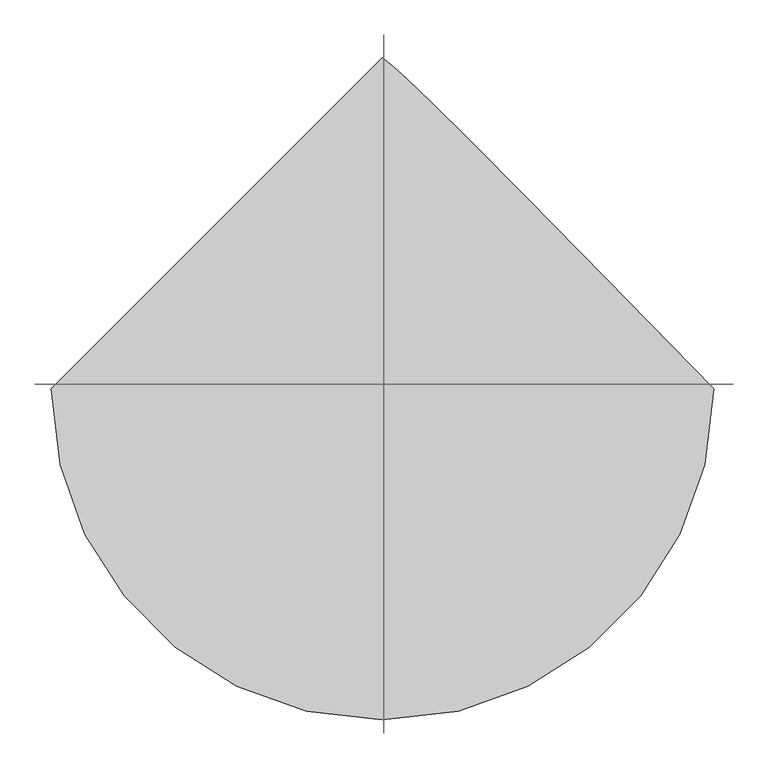
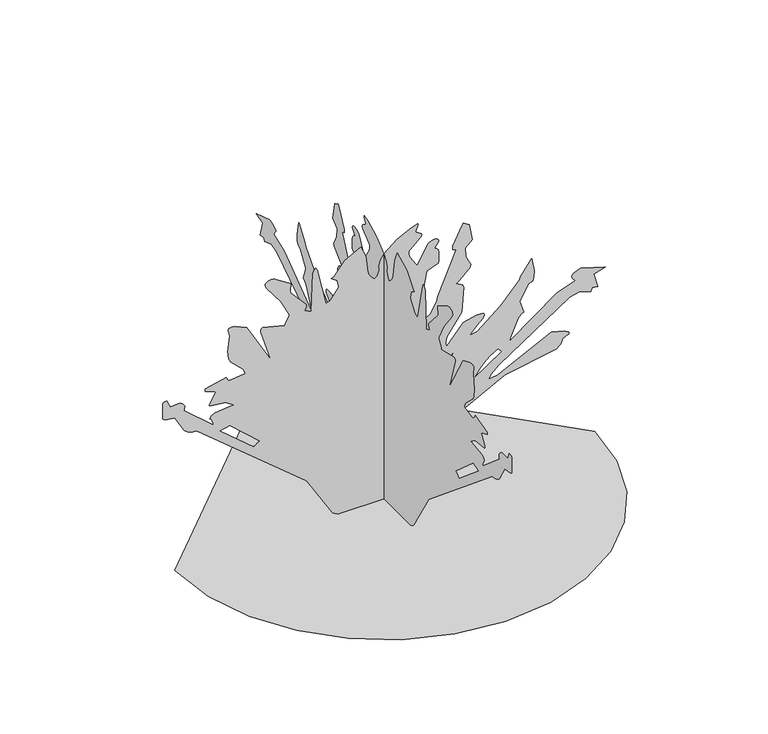
"""IFC4 building model written with IfcOpenShell, lengths in millimetres: proxy geometry, prairie dropseed 26760 : prairie dropseed 26760."""

import ifcopenshell
import ifcopenshell.guid

model = None  # the IFC model being written
_history = None  # IfcOwnerHistory: only IFC2X3 demands one
_inside = {}  # id of a spatial element -> (the spatial element, [elements in it])
_under = {}  # id of a project, library or spatial element -> (it, [spatial elements below it])
_declared = {}  # id of a project -> (the project, [libraries it declares])
_typed = {}  # id of a type object -> (the type object, [elements of that type])
_made_of = {}  # id of a material, layer set ... -> (it, [elements and type objects made of it])


def new_model(schema):
    """Start an empty IFC model of exactly this schema.

    Asked for "IFC4X3", IfcOpenShell would pick the latest addendum, in which some entities
    have other attributes; the version numbers below select the first issue.
    IFC2X3 requires an IfcOwnerHistory on every rooted entity: one is made here for all.
    """
    global model, _history
    if schema == "IFC4X3":
        model = ifcopenshell.file(schema_version=(4, 3, 0, 0))
    else:
        model = ifcopenshell.file(schema=schema)
    _inside.clear()
    _under.clear()
    _declared.clear()
    _typed.clear()
    _made_of.clear()
    _history = None
    if model.schema == "IFC2X3":
        org = make("IfcOrganization", Name="unknown")
        user = make(
            "IfcPersonAndOrganization",
            ThePerson=make("IfcPerson", FamilyName="unknown"),
            TheOrganization=org,
        )
        app = make(
            "IfcApplication",
            ApplicationDeveloper=org,
            Version="unknown",
            ApplicationFullName="unknown",
            ApplicationIdentifier="unknown",
        )
        _history = make(
            "IfcOwnerHistory",
            OwningUser=user,
            OwningApplication=app,
            ChangeAction="ADDED",
            CreationDate=0,
        )
    return model


def make(cls, **values):
    """One entity of the class cls with the attributes given. An attribute that is None is left unset."""
    return model.create_entity(
        cls, **{name: value for name, value in values.items() if value is not None}
    )


def rooted(cls, **values):
    """An entity with a GlobalId (a new one), such as an element, a storey or a relation."""
    return make(cls, GlobalId=ifcopenshell.guid.new(), OwnerHistory=_history, **values)


def si_unit(unit_type, name, prefix=None):
    """IfcSIUnit, for example si_unit("LENGTHUNIT", "METRE", prefix="MILLI")."""
    return make("IfcSIUnit", UnitType=unit_type, Prefix=prefix, Name=name)


def assignment(units):
    """IfcUnitAssignment: the units of a project."""
    return None if units is None else make("IfcUnitAssignment", Units=units)


def point(xyz):
    """IfcCartesianPoint."""
    return None if xyz is None else make("IfcCartesianPoint", Coordinates=xyz)


def direction(xyz):
    """IfcDirection."""
    return None if xyz is None else make("IfcDirection", DirectionRatios=xyz)


def frame(location, z_axis=None, x_axis=None):
    """IfcAxis2Placement3D, a coordinate frame: its origin and axes. An axis left out is left unset."""
    return make(
        "IfcAxis2Placement3D",
        Location=point(location),
        Axis=direction(z_axis),
        RefDirection=direction(x_axis),
    )


def origin():
    """The frame at (0, 0, 0) with its axes left unset."""
    return frame((0.0, 0.0, 0.0))


def place(relative_to, where):
    """IfcLocalPlacement: puts the frame where relative to a parent placement (None: the world)."""
    return make(
        "IfcLocalPlacement", PlacementRelTo=relative_to, RelativePlacement=where
    )


def context(
    kind, dimensions, precision=None, world=None, true_north=None, identifier=None
):
    """IfcGeometricRepresentationContext, for example the 3D "Model" context."""
    return make(
        "IfcGeometricRepresentationContext",
        ContextIdentifier=identifier,
        ContextType=kind,
        CoordinateSpaceDimension=dimensions,
        Precision=precision,
        WorldCoordinateSystem=world,
        TrueNorth=true_north,
    )


def project(units=None, contexts=None):
    """IfcProject with its units and contexts."""
    return rooted(
        "IfcProject",
        Name="project",
        RepresentationContexts=contexts,
        UnitsInContext=assignment(units),
    )


def spatial(cls, under=None, at=None, **own):
    """A site, building, storey or space (cls), placed at a placement, below another one or the project."""
    s = rooted(cls, ObjectPlacement=at, **own)
    if under is not None:
        _under.setdefault(under.id(), (under, []))[1].append(s)
    return s


def point_list(points):
    """IfcCartesianPointList2D or 3D."""
    cls = (
        "IfcCartesianPointList2D" if len(points[0]) == 2 else "IfcCartesianPointList3D"
    )
    return make(cls, CoordList=points)


def triangles(points, corners, closed=None, point_numbers=None):
    """IfcTriangulatedFaceSet: each triangle names its three corners, points numbered from 1."""
    return make(
        "IfcTriangulatedFaceSet",
        Coordinates=point_list(points),
        Closed=closed,
        CoordIndex=corners,
        PnIndex=point_numbers,
    )


def shape(context_of_items, identifier, shape_type, items):
    """IfcShapeRepresentation: the items that make up one representation, for example the "Body"."""
    return make(
        "IfcShapeRepresentation",
        ContextOfItems=context_of_items,
        RepresentationIdentifier=identifier,
        RepresentationType=shape_type,
        Items=items,
    )


def source(mapping_origin, context_of_items, identifier, shape_type, items):
    """IfcRepresentationMap: a shape defined once, which mapped items show again and again."""
    return make(
        "IfcRepresentationMap",
        MappingOrigin=mapping_origin,
        MappedRepresentation=shape(context_of_items, identifier, shape_type, items),
    )


def transform(
    local_origin,
    x_axis=None,
    y_axis=None,
    z_axis=None,
    scale=None,
    scale2=None,
    scale3=None,
    uniform=True,
):
    """IfcCartesianTransformationOperator3D, or its non-uniform kind. x_axis, y_axis, z_axis: its Axis1, 2, 3."""
    if uniform:
        return make(
            "IfcCartesianTransformationOperator3D",
            Axis1=direction(x_axis),
            Axis2=direction(y_axis),
            LocalOrigin=point(local_origin),
            Scale=scale,
            Axis3=direction(z_axis),
        )
    return make(
        "IfcCartesianTransformationOperator3DnonUniform",
        Axis1=direction(x_axis),
        Axis2=direction(y_axis),
        LocalOrigin=point(local_origin),
        Scale=scale,
        Axis3=direction(z_axis),
        Scale2=scale2,
        Scale3=scale3,
    )


def mapped(mapping_source, mapping_target):
    """IfcMappedItem: shows the shape of a source again, moved by a transform."""
    return make(
        "IfcMappedItem", MappingSource=mapping_source, MappingTarget=mapping_target
    )


def made_of(thing, what):
    """Note that an element or type object is made of a material, layer set ...; save() writes the relation."""
    if what is not None:
        _made_of.setdefault(what.id(), (what, []))[1].append(thing)
    return thing


def element(
    cls,
    number,
    at=None,
    inside=None,
    cuts=None,
    type_object=None,
    material=None,
    context=None,
    identifier="Body",
    shape_type=None,
    held_by="IfcProductDefinitionShape",
    body=None,
    shapes=None,
    **own,
):
    """One element of the class cls, such as IfcWall. Its Tag is "e" and its number.

    at: its placement. inside: the storey or other place that contains it. cuts: it is an
    opening in that element (IfcRelVoidsElement). A single representation is given by context,
    identifier, shape_type and body (its items); several are given by shapes. held_by: the class
    of the entity that holds the representations. save() writes the other relations.
    """
    e = rooted(cls, Tag="e%d" % number, ObjectPlacement=at, **own)
    if body is not None:
        shapes = [shape(context, identifier, shape_type, body)]
    if shapes is not None:
        e.Representation = make(held_by, Representations=shapes)
    if inside is not None:
        _inside.setdefault(inside.id(), (inside, []))[1].append(e)
    if cuts is not None:
        rooted(
            "IfcRelVoidsElement", RelatingBuildingElement=cuts, RelatedOpeningElement=e
        )
    if type_object is not None:
        _typed.setdefault(type_object.id(), (type_object, []))[1].append(e)
    return made_of(e, material)


def aggregate(whole, parts):
    """IfcRelAggregates: a whole, such as a stair, and the parts it consists of."""
    return rooted("IfcRelAggregates", RelatingObject=whole, RelatedObjects=parts)


def save(model, path):
    """Write the relations noted so far, then the file.

    IfcRelAggregates (storeys below a building ...), IfcRelContainedInSpatialStructure (elements
    in a storey), IfcRelDefinesByType, IfcRelAssociatesMaterial and IfcRelDeclares: one each for
    every whole, place, type object, material and project.
    """
    for whole, parts in _under.values():
        aggregate(whole, parts)
    for where, things in _inside.values():
        rooted(
            "IfcRelContainedInSpatialStructure",
            RelatedElements=things,
            RelatingStructure=where,
        )
    for kind, things in _typed.values():
        rooted("IfcRelDefinesByType", RelatedObjects=things, RelatingType=kind)
    for what, things in _made_of.values():
        rooted("IfcRelAssociatesMaterial", RelatedObjects=things, RelatingMaterial=what)
    for by, libraries in _declared.values():
        rooted("IfcRelDeclares", RelatingContext=by, RelatedDefinitions=libraries)
    model.write(path)


def entourage_02fa341a(model_context):
    return source(origin(), model_context, "Body", "Tessellation", [
        triangles([(-1145.8724991, 0.0, 0.0001203), (-1115.5778366, -262.5577928, 0.0001203), (-1029.3040329, -503.6753972, 0.0001203), (-893.9573524, -716.4439871, 0.0001203), (-716.4439871, -893.9573524, 0.0001203), (-503.6753972, -1029.3040329, 0.0001203), (-262.5577928, -1115.5778366, 0.0001203), (5.01e-05, -1145.8724991, 0.0001203), (262.5577928, -1115.5778366, 0.0001203), (503.6753972, -1029.3040329, 0.0001203), (716.4439871, -893.9573524, 0.0001203), (893.9573524, -716.4439871, 0.0001203), (1029.3040329, -503.6753972, 0.0001203), (1115.5778366, -262.5577928, 0.0001203), (1145.8724991, 0.0001002, 0.0001203), (773.4874529, 381.9735961, 0.0001203), (497.4218908, 663.2029781, 0.0001203), (301.6205247, 860.4800354, 0.0001203), (170.0304827, 990.5943317, 0.0001203), (86.5989292, 1070.3377928, 0.0001203), (35.272797, 1116.4998734, 0.0001203), (-0.0001503, 1145.8724991, 0.0001203), (191.5793673, 16.4808481, 1518.7299728), (190.2057411, 16.4808481, 1512.532386), (177.5557501, 16.4808481, 1485.8293648), (178.0462362, 16.4808481, 1480.5131195), (207.8564987, 16.4808481, 1461.7196445), (211.32233, 16.4808481, 1451.7881287), (204.1071818, 16.4808481, 1439.5808796), (144.6111222, 16.4808481, 1389.2583698), (141.1229358, 16.4808481, 1381.6383408), (140.426721, 16.4808481, 1366.2256187), (146.0929631, 16.4808481, 1347.6911396), (178.4658327, 16.4808481, 1296.2230602), (186.7823127, 16.4808481, 1288.0619305), (190.0609643, 16.4808481, 1288.211776), (245.3213086, 16.4808481, 1386.9849621), (252.3454438, 16.4808481, 1394.9860725), (265.8470906, 16.4808481, 1400.4698948), (281.8237317, 16.4808481, 1402.5959278), (289.4335869, 16.4808481, 1401.7577522), (296.0960073, 16.4808481, 1399.3065937), (301.2827002, 16.4808481, 1394.9860725), (303.525532, 16.4808481, 1388.0517574), (301.6992627, 16.4808481, 1380.2565937), (279.0398718, 16.4808481, 1350.4953289), (292.1132926, 16.4808481, 1346.2916611), (300.5334, 16.4808481, 1335.2070179), (305.1155694, 16.4808481, 1319.5453285), (303.9395511, 16.4808481, 1268.0670753), (301.2827002, 16.4808481, 1257.0687641), (238.9982207, 16.4808481, 1234.823465), (219.7373687, 16.4808742, 1135.2349216), (208.8420127, 16.4808742, 1067.5641249), (212.3832936, 16.4808742, 1036.2585503), (225.652015, 16.4808742, 1007.9299015), (234.5499094, 16.4808742, 967.8917931), (248.2595922, 16.4808742, 970.7670536), (258.6512544, 16.4808742, 978.4505962), (292.3850601, 16.4808742, 1039.0729134), (298.2194605, 16.4808742, 1065.3949986), (399.1592477, 16.4808481, 1301.557037), (381.5697327, 16.4808481, 1309.1974136), (379.2862601, 16.4808481, 1328.9001354), (432.7863739, 16.4808481, 1431.8338234), (439.1998996, 16.4808481, 1439.4742001), (469.1567193, 16.4808481, 1422.9108215), (470.340368, 16.4808481, 1421.67892), (488.1381915, 16.4808481, 1328.2525005), (448.0975396, 16.4808481, 1292.6593243), (452.5450879, 16.4808481, 1243.7211777), (475.4661089, 16.4808742, 1195.1663652), (479.2405515, 16.4808742, 1190.3352648), (474.884422, 16.4808742, 1175.0165051), (415.7048584, 16.4808742, 1116.6548058), (399.1592477, 16.4808742, 1105.8064854), (400.510546, 16.4808742, 1104.4069342), (434.7498078, 16.4808742, 1083.5611135), (441.3436641, 16.4808742, 1069.7841202), (428.4937943, 16.4808742, 930.2133516), (347.4472878, 16.4808992, 815.783563), (341.366518, 16.4808992, 788.9789492), (345.7734438, 16.4808992, 758.7935097), (439.1998996, 16.4808742, 865.5651175), (512.8727283, 16.4808742, 883.5687424), (542.821954, 16.4808742, 883.172473), (547.2034452, 16.4808742, 881.851696), (550.2463918, 16.4808742, 879.4843987), (551.976119, 16.4808742, 876.1493551), (552.4231484, 16.4808742, 871.9304266), (551.610371, 16.4808742, 866.9087854), (549.5681992, 16.4808742, 861.1709089), (543.2842441, 16.4808742, 853.7287033), (531.917714, 16.4808742, 842.4993742), (517.6733437, 16.4808992, 828.930653), (502.7584474, 16.4808992, 814.4704165), (489.3751436, 16.4808992, 800.5638525), (479.7282034, 16.4808992, 788.6613813), (476.0198178, 16.4808992, 780.210807), (513.8201632, 16.4808992, 789.5783312), (642.9667133, 16.4808742, 892.3291815), (746.172187, 16.4808742, 1007.9299015), (749.7891901, 16.4808742, 1021.8363928), (808.727453, 16.4808742, 1102.2682566), (812.905759, 16.4808742, 1105.8064854), (824.3001944, 16.4808742, 1031.1582075), (823.6322119, 16.4808742, 994.8412382), (817.3558508, 16.4808742, 972.3393414), (795.110479, 16.4808742, 967.8917931), (747.0028049, 16.4808742, 882.9210348), (746.172187, 16.4808742, 878.9128492), (768.4175589, 16.4808992, 812.1793499), (753.3274189, 16.4808992, 805.8165842), (738.2855318, 16.4808992, 789.0373032), (695.1587311, 16.4808992, 686.8503719), (692.7864195, 16.4808992, 669.8145658), (947.0688635, 16.4808742, 860.4216087), (1048.699506, 16.4808742, 896.7081293), (1031.5646507, 16.4808742, 917.3609385), (1030.2641487, 16.4808742, 922.2631102), (1030.9016825, 16.4808742, 927.8511412), (1034.3306883, 16.4808742, 934.1604944), (1040.9118273, 16.4808742, 940.3403498), (1059.8323294, 16.4808742, 950.6222803), (1080.2666925, 16.4808742, 955.3314405), (1088.7376144, 16.4808742, 954.5440613), (1213.3071184, 16.4808742, 914.5034094), (1151.0236382, 16.4808742, 896.7081293), (1173.2664665, 16.4808992, 816.6268982), (1142.1259981, 16.4808992, 821.0769899), (1133.2283581, 16.4808992, 803.2817099), (1073.0276722, 16.4808742, 824.1351608), (1018.2448242, 16.4808992, 810.9525352), (631.9609171, 16.4808992, 554.5135732), (591.7932381, 16.4808992, 516.5074991), (577.1145555, 16.4808992, 491.8592943), (627.4016024, 16.4808992, 498.6258508), (914.8336218, 16.4808992, 642.3291796), (919.6799829, 16.4808992, 643.1216457), (989.570775, 16.4808992, 625.9969643), (1013.5077587, 16.4808992, 611.3792519), (1017.1018707, 16.4808992, 604.5339211), (1013.9115858, 16.4808992, 600.0584312), (1009.2633957, 16.4808992, 596.634476), (980.9245731, 16.4808992, 585.3568577), (971.1252439, 16.4808992, 556.8427915), (945.85215, 16.4808992, 537.2669515), (663.4595032, 16.4808992, 486.10365), (303.2308916, 16.4809242, 297.9146645), (169.4772643, 16.4809242, 161.3263992), (69.2098062, 16.4809242, 12.9610616), (67.9149089, 16.4809242, 9.6154435), (64.4996195, 16.4809242, 6.7499111), (47.3677937, 16.4809242, 1.1487808), (-237.5664222, 16.4809242, 3.55e-05), (-244.2689927, 16.4809242, 1.6405105), (-251.0271739, 16.4809242, 4.0836423), (-257.5565174, 16.4809242, 7.0952757), (-263.5737918, 16.4809242, 10.4413515), (-268.793495, 16.4809242, 13.8879604), (-272.9311604, 16.4809242, 17.2006602), (-275.702303, 16.4809242, 20.1455931), (-415.6845471, 16.4809242, 251.3398547), (-1015.5905531, 16.4808992, 749.8933262), (-1043.5331789, 16.4808992, 753.4493591), (-1066.7030582, 16.4808992, 763.3172161), (-1085.8064707, 16.4808992, 778.3058361), (-1135.7099653, 16.4808742, 865.5651175), (-1188.5954, 16.4808742, 874.7803253), (-1197.2085371, 16.4808742, 878.409973), (-1202.4434647, 16.4808742, 883.3603975), (-1200.9524946, 16.4808742, 970.6299253), (-1197.9959164, 16.4808742, 976.7894331), (-1180.2006363, 16.4808742, 981.2369814), (-1162.4053562, 16.4808742, 941.1963295), (-1112.0319775, 16.4808742, 943.6424011), (-1102.0192892, 16.4808742, 939.9618845), (-1092.2453945, 16.4808742, 932.1361267), (-1082.3241251, 16.4808742, 918.9535011), (-1086.0451916, 16.4808742, 894.3433754), (-1086.7716734, 16.4808742, 892.2580376), (-926.6116093, 16.4808992, 754.3434179), (-925.605784, 16.4808992, 759.362443), (-927.0764791, 16.4808992, 766.1722017), (-938.5826809, 16.4808992, 788.0010292), (-942.1971405, 16.4808992, 792.6314152), (-944.4068893, 16.4808992, 794.3840698), (-937.4142929, 16.4808992, 808.8823854), (-919.3421402, 16.4808992, 818.6817146), (-823.4569319, 16.4808742, 829.6215265), (-815.3899097, 16.4808742, 829.97463), (-858.7680759, 16.4808742, 860.6984814), (-944.4068893, 16.4808742, 870.0152092), (-947.1628258, 16.4808742, 873.2892826), (-945.4203449, 16.4808742, 881.8338919), (-918.6309191, 16.4808742, 930.5131153), (-913.2664209, 16.4808742, 936.7487812), (-916.3169615, 16.4808742, 939.0652822), (-971.1023529, 16.4808742, 963.4417013), (-971.1023529, 16.4808742, 976.7894331), (-855.4305616, 16.4808742, 1003.4823532), (-846.5329216, 16.4808742, 985.6870731), (-841.8745577, 16.4808742, 979.8552343), (-829.7383799, 16.4808742, 977.9705383), (-753.1064295, 16.4808742, 990.1346214), (-756.4770086, 16.4808742, 1006.0553793), (-765.4127277, 16.4808742, 1020.5536949), (-831.3791954, 16.4808742, 1083.2842409), (-840.7899582, 16.4808742, 1103.5102592), (-847.4701464, 16.4808742, 1148.4429817), (-835.9664881, 16.4808481, 1236.4922585), (-844.9453732, 16.4808481, 1268.2270947), (-844.5237419, 16.4808481, 1274.356081), (-842.0828299, 16.4808481, 1279.3142086), (-823.4467581, 16.4808481, 1281.6536007), (-807.3482494, 16.4808481, 1280.2336292), (-744.2087894, 16.4808481, 1252.618745), (-611.5748068, 16.4808742, 1020.9982172), (-667.4397108, 16.4808742, 1200.5004147), (-666.7716557, 16.4808742, 1209.9873356), (-663.0404154, 16.4808742, 1217.4803375), (-655.2298456, 16.4808742, 1221.4783493), (-535.1105061, 16.4808742, 1190.3352648), (-533.8786045, 16.4808742, 1199.9263218), (-512.8651342, 16.4808481, 1239.2736294), (-511.3157375, 16.4808481, 1244.1986195), (-557.3532981, 16.4808481, 1337.1500679), (-634.6126448, 16.4808481, 1439.0804741), (-643.7160135, 16.4808481, 1457.800407), (-641.8821138, 16.4808481, 1466.1671928), (-637.6073021, 16.4808481, 1471.8948956), (-632.047249, 16.4808481, 1476.1239979), (-625.5575289, 16.4808481, 1478.9915554), (-611.2090588, 16.4808481, 1481.1760151), (-597.39395, 16.4808481, 1479.5149246), (-503.9674942, 16.4808481, 1421.67892), (-502.3393596, 16.4808481, 1414.2646923), (-507.1602862, 16.4808481, 1383.6296436), (-506.7665603, 16.4808481, 1375.9283695), (-503.9674942, 16.4808481, 1368.290609), (-419.4386421, 16.4808481, 1270.4164959), (-417.9679833, 16.4808481, 1265.4483398), (-418.4759829, 16.4808481, 1259.8959171), (-428.3362822, 16.4808481, 1239.2736294), (-392.7457583, 16.4808742, 1221.4783493), (-382.6517524, 16.4808481, 1438.78587), (-376.0604396, 16.4808481, 1454.3636982), (-366.0502948, 16.4808481, 1461.7196445), (-358.5369452, 16.4808481, 1448.6461693), (-312.6644546, 16.4808481, 1243.7211777), (-312.6644546, 16.4808481, 1239.2736294), (-297.8790925, 16.4808481, 1242.0853764), (-285.9918639, 16.4808481, 1249.6164574), (-241.4823532, 16.4808481, 1310.4546043), (-250.3804838, 16.4808481, 1350.4953289), (-281.5214609, 16.4808481, 1372.7406281), (-269.5834359, 16.4808481, 1376.9621727), (-207.497836, 16.4808481, 1449.829818), (-121.3619509, 16.4808481, 1497.3102047), (-95.2247926, 16.4808481, 1437.6657349), (-83.2026885, 16.4808481, 1344.1731857), (-76.9446311, 16.4808481, 1324.6506855), (-65.1584955, 16.4808481, 1306.0909172), (-45.7307615, 16.4808481, 1288.211776), (-41.5217161, 16.4808481, 1290.5004444), (-35.9095768, 16.4808481, 1296.6929443), (-29.9423425, 16.4808481, 1305.7657917), (-24.6679461, 16.4808481, 1316.7005894), (-21.135356, 16.4808481, 1328.4811203), (-20.392126, 16.4808481, 1340.0863712), (-23.4862072, 16.4808481, 1350.4953289), (-15.2394211, 16.4808481, 1383.2867867), (6.9086104, 16.4808481, 1415.9385727), (77.353318, 16.4808481, 1474.7548954), (156.7378711, 16.4808481, 1514.8082645), (190.0609643, 16.4808481, 1524.0030521), (314.8691892, 16.4808992, 650.9652077), (302.783844, 16.4808992, 632.2733253), (297.6250927, 16.4808992, 615.8852268), (301.2827002, 16.4808992, 603.0810302), (316.0884098, 16.4808992, 608.5598019), (394.7091559, 16.4808992, 723.2004061), (-891.0210491, 16.4808992, 705.405126), (-704.1681376, 16.4808992, 549.69519), (-701.9100632, 16.4808992, 552.6847967), (-698.0060863, 16.4808992, 556.3906388), (-693.0047928, 16.4808992, 560.4190993), (-687.457457, 16.4808992, 564.3789594), (-681.9125919, 16.4808992, 567.8816525), (-676.9164579, 16.4808992, 570.5308731), (-673.0251257, 16.4808992, 571.9380183), (-837.6352816, 16.4808992, 718.7528578), (585.3822558, 16.4808992, 625.1511583), (564.2392513, 16.4808992, 606.7843652), (544.2418164, 16.4808992, 586.416059), (525.5346734, 16.4808992, 565.0190366), (508.2651607, 16.4808992, 543.5585369), (492.5857398, 16.4808992, 522.9997627), (648.2982193, 16.4808992, 625.3263657), (630.5029392, 16.4808992, 647.569194), (630.5029392, 16.4808992, 652.0192858), (5.4318519, 202.6286565, 1518.7299728), (5.4318519, 201.2550121, 1512.532386), (5.4318519, 188.6050212, 1485.8293648), (5.4318519, 189.0955072, 1480.5131195), (5.4318519, 218.9057698, 1461.7196445), (5.4318519, 222.3716011, 1451.7881287), (5.4318519, 215.156471, 1439.5808796), (5.4318519, 155.6603933, 1389.2583698), (5.4318519, 152.1722159, 1381.6383408), (5.4318519, 151.4760012, 1366.2256187), (5.4318519, 157.1419889, 1347.6911396), (5.4318519, 189.5151219, 1296.2230602), (5.4318519, 197.8316019, 1288.0619305), (5.4318519, 201.1102354, 1288.211776), (5.4318519, 256.3703253, 1386.9849621), (5.4318519, 263.3959866, 1394.9860725), (5.4318519, 276.8961073, 1400.4698948), (5.4318519, 292.8752918, 1402.5959278), (5.4318519, 300.4826036, 1401.7577522), (5.4318519, 307.145024, 1399.3065937), (5.4318519, 312.331735, 1394.9860725), (5.4318519, 314.5745487, 1388.0517574), (5.4318519, 312.7482794, 1380.2565937), (5.4318519, 290.0889067, 1350.4953289), (5.4318519, 303.1623093, 1346.2916611), (5.4318519, 311.5824348, 1335.2094887), (5.4318519, 316.1646043, 1319.5453285), (5.4318519, 314.9885859, 1268.0670753), (5.4318519, 312.331735, 1257.0687641), (5.4318519, 250.0474917, 1234.823465), (5.4318519, 230.7866398, 1135.2349216), (5.4318519, 219.8912838, 1067.5641249), (5.4318519, 223.4325647, 1036.2585503), (5.4318519, 236.7015404, 1007.9299015), (5.4318519, 245.5991804, 967.8917931), (5.4318519, 259.3091176, 970.7695971), (5.4318519, 269.7002711, 978.4531397), (5.4318519, 303.434095, 1039.0729134), (5.4318519, 309.2684772, 1065.3949986), (5.4318519, 410.2082826, 1301.557037), (5.4318519, 392.6187312, 1309.1974136), (5.4318519, 390.3378385, 1328.9001354), (5.4318519, 443.8354088, 1431.8338234), (5.4318519, 450.2489345, 1439.4742001), (5.4318519, 480.2057542, 1422.9108215), (5.4318519, 481.39191, 1421.67892), (5.4318519, 499.1871901, 1328.2525005), (5.4318519, 459.1465745, 1292.6593243), (5.4318519, 463.5941228, 1243.7236485), (5.4318519, 486.5151074, 1195.1663652), (5.4318519, 490.28955, 1190.3352648), (5.4318519, 485.9334569, 1175.0165051), (5.4318519, 426.7538569, 1116.6548058), (5.4318519, 410.2082826, 1105.8064854), (5.4318519, 411.5595809, 1104.4069342), (5.4318519, 445.7988427, 1083.5611135), (5.4318519, 452.392699, 1069.7841202), (5.4318519, 439.5427929, 930.2133516), (5.4318519, 358.4963227, 815.783563), (5.4318519, 352.4155529, 788.9789492), (5.4318519, 356.8224423, 758.7935097), (5.4318519, 450.2489345, 865.5651175), (5.4318519, 523.9217631, 883.5687424), (5.4318519, 553.8709525, 883.172473), (5.4318519, 558.2524801, 881.8542395), (5.4318519, 561.2953903, 879.4843987), (5.4318519, 563.0251539, 876.1493551), (5.4318519, 563.4721833, 871.9304266), (5.4318519, 562.6593696, 866.9087854), (5.4318519, 560.617234, 861.1709089), (5.4318519, 554.3332426, 853.7287033), (5.4318519, 542.9667126, 842.4993742), (5.4318519, 528.7223785, 828.930653), (5.4318519, 513.8074822, 814.4704165), (5.4318519, 500.4241785, 800.5638525), (5.4318519, 490.7772383, 788.6613813), (5.4318519, 487.0688164, 780.210807), (5.4318519, 524.869198, 789.5783312), (5.4318519, 654.0157482, 892.3291815), (5.4318519, 757.2237654, 1007.9299015), (5.4318519, 760.838225, 1021.8363928), (5.4318519, 819.7790314, 1102.2682566), (5.4318519, 823.9547939, 1105.8064854), (5.4318519, 835.3517727, 1031.1582075), (5.4318519, 834.6812468, 994.8412382), (5.4318519, 828.4048857, 972.3393414), (5.4318519, 806.1595139, 967.8917931), (5.4318519, 758.0518398, 882.9210348), (5.4318519, 757.2237654, 878.9128492), (5.4318519, 779.4665937, 812.1793499), (5.4318519, 764.3764538, 805.8191277), (5.4318519, 749.334494, 789.0373032), (5.4318519, 706.207766, 686.8503719), (5.4318519, 703.8353817, 669.8145658), (5.4318519, 958.1178257, 860.4216087), (5.4318519, 1059.7485409, 896.7081293), (5.4318519, 1042.6162291, 917.3609385), (5.4318519, 1041.3131836, 922.2631102), (5.4318519, 1041.9532608, 927.8511412), (5.4318519, 1045.3797232, 934.1604944), (5.4318519, 1051.9608622, 940.3403498), (5.4318519, 1070.8813643, 950.6222803), (5.4318519, 1091.3157274, 955.3314405), (5.4318519, 1099.7866493, 954.5440613), (5.4318519, 1224.3560806, 914.5034094), (5.4318519, 1162.072673, 896.7081293), (5.4318519, 1184.3155014, 816.6268982), (5.4318519, 1153.175033, 821.0769899), (5.4318519, 1144.277393, 803.2817099), (5.4318519, 1084.0767071, 824.1351608), (5.4318519, 1029.2938591, 810.9525352), (5.4318519, 643.0098793, 554.5135732), (5.4318519, 602.8422729, 516.5074991), (5.4318519, 588.1635904, 491.8592943), (5.4318519, 638.4505646, 498.6258508), (5.4318519, 925.8826567, 642.3291796), (5.4318519, 930.7289452, 643.1216457), (5.4318519, 1000.6197372, 625.9969643), (5.4318519, 1024.5567936, 611.3792519), (5.4318519, 1028.1509056, 604.5339211), (5.4318519, 1024.9606207, 600.0584312), (5.4318519, 1020.314974, 596.634476), (5.4318519, 991.9761515, 585.3568577), (5.4318519, 982.1742788, 556.8427915), (5.4318519, 956.9011848, 537.2669515), (5.4318519, 674.5085381, 486.10365), (5.4318519, 314.2799083, 297.9146645), (5.4318519, 180.5265354, 161.3261448), (5.4318519, 80.2590818, 12.9610366), (5.4318519, 78.9641845, 9.6153924), (5.4318519, 75.5488951, 6.7498855), (5.4318519, 58.4170693, 1.1487452), (5.4318519, -226.5171511, 0.0), (5.4318519, -233.2197035, 1.640475), (5.4318519, -239.9779029, 4.0835915), (5.4318519, -246.5075007, 7.0952502), (5.4318519, -252.5237577, 10.4413253), (5.4318519, -257.7419349, 13.8879093), (5.4318519, -261.8821436, 17.2006352), (5.4318519, -264.6532863, 20.1455681), (5.4318519, -404.6355123, 251.3398547), (5.4318519, -1004.5415182, 749.8933262), (5.4318519, -1032.484144, 753.4493591), (5.4318519, -1055.6540234, 763.3172161), (5.4318519, -1074.7574358, 778.3058361), (5.4318519, -1124.6609304, 865.5651175), (5.4318519, -1177.5463652, 874.7803253), (5.4318519, -1186.1595022, 878.409973), (5.4318519, -1191.3944298, 883.3603975), (5.4318519, -1189.9034597, 970.6299253), (5.4318519, -1186.9468815, 976.7894331), (5.4318519, -1169.1516741, 981.2369814), (5.4318519, -1151.356394, 941.1963295), (5.4318519, -1100.9830153, 943.6424011), (5.4318519, -1090.9702543, 939.9618845), (5.4318519, -1081.1963596, 932.1361267), (5.4318519, -1071.2750902, 918.9535011), (5.4318519, -1074.9961567, 894.3433754), (5.4318519, -1075.7226385, 892.260581), (5.4318519, -915.5626471, 754.3434179), (5.4318519, -914.5567492, 759.362443), (5.4318519, -916.0274443, 766.1722017), (5.4318519, -927.533646, 788.0010292), (5.4318519, -931.1481056, 792.6314152), (5.4318519, -933.3578545, 794.3840698), (5.4318519, -926.365258, 808.8823854), (5.4318519, -908.2905619, 818.6817146), (5.4318519, -812.407897, 829.62407), (5.4318519, -804.3408749, 829.97463), (5.4318519, -847.7165703, 860.6984814), (5.4318519, -933.3578545, 870.0152092), (5.4318519, -936.1137909, 873.2892826), (5.4318519, -934.3713827, 881.8338919), (5.4318519, -907.5818842, 930.5131153), (5.4318519, -902.2174587, 936.7487812), (5.4318519, -905.2679993, 939.0652822), (5.4318519, -960.053318, 963.4417013), (5.4318519, -960.053318, 976.7894331), (5.4318519, -844.3815268, 1003.4823532), (5.4318519, -835.4838867, 985.6870731), (5.4318519, -830.8255228, 979.8552343), (5.4318519, -818.6868015, 977.9705383), (5.4318519, -742.0573946, 990.1346214), (5.4318519, -745.4279737, 1006.0553793), (5.4318519, -754.3636929, 1020.5536949), (5.4318519, -820.3302332, 1083.2842409), (5.4318519, -829.7409233, 1103.5102592), (5.4318519, -836.4211115, 1148.4429817), (5.4318519, -824.9174532, 1236.4922585), (5.4318519, -833.8963383, 1268.2270947), (5.4318519, -833.474707, 1274.356081), (5.4318519, -831.033795, 1279.3142086), (5.4318519, -812.3977959, 1281.6536007), (5.4318519, -796.2992146, 1280.2336292), (5.4318519, -733.1597546, 1252.6212158), (5.4318519, -600.5257719, 1020.9982172), (5.4318519, -656.3906759, 1200.5004147), (5.4318519, -655.7226208, 1209.9873356), (5.4318519, -651.9913805, 1217.4803375), (5.4318519, -644.1808834, 1221.4783493), (5.4318519, -524.0614712, 1190.3352648), (5.4318519, -522.8270262, 1199.9263218), (5.4318519, -501.8160994, 1239.2736294), (5.4318519, -500.2667027, 1244.1986195), (5.4318519, -546.3042995, 1337.1500679), (5.4318519, -623.5636099, 1439.0804741), (5.4318519, -632.6669786, 1457.800407), (5.4318519, -630.8331516, 1466.1671928), (5.4318519, -626.5582672, 1471.8948956), (5.4318519, -620.9982141, 1476.1239979), (5.4318519, -614.508494, 1478.9915554), (5.4318519, -600.1600239, 1481.1760151), (5.4318519, -586.3449151, 1479.5149246), (5.4318519, -492.9184593, 1421.67892), (5.4318519, -491.2903247, 1414.2646923), (5.4318519, -496.1087079, 1383.6296436), (5.4318519, -495.7175617, 1375.9283695), (5.4318519, -492.9184593, 1368.290609), (5.4318519, -408.3896436, 1270.4164959), (5.4318519, -406.9189848, 1265.4483398), (5.4318519, -407.4269843, 1259.8959171), (5.4318519, -417.2872836, 1239.2736294), (5.4318519, -381.6967235, 1221.4783493), (5.4318519, -371.6027538, 1438.78587), (5.4318519, -365.011441, 1454.3636982), (5.4318519, -355.0012599, 1461.7196445), (5.4318519, -347.4854033, 1448.6487854), (5.4318519, -301.6154378, 1243.7236485), (5.4318519, -301.6154378, 1239.2736294), (5.4318519, -286.8300758, 1242.0853764), (5.4318519, -274.9428472, 1249.6164574), (5.4318519, -230.433064, 1310.4546043), (5.4318519, -239.3312127, 1350.4953289), (5.4318519, -270.4724442, 1372.7406281), (5.4318519, -258.5318758, 1376.9621727), (5.4318519, -196.448565, 1449.829818), (5.4318519, -110.3126707, 1497.3102047), (5.4318519, -84.1755125, 1437.6657349), (5.4318519, -72.1534174, 1344.1731857), (5.4318519, -65.895351, 1324.6506855), (5.4318519, -54.1092199, 1306.0909172), (5.4318519, -34.6814836, 1288.211776), (5.4318519, -30.4726948, 1290.5004444), (5.4318519, -24.860274, 1296.6929443), (5.4318519, -18.8929897, 1305.7657917), (5.4318519, -13.6186943, 1316.7005894), (5.4318519, -10.0861065, 1328.4811203), (5.4318519, -9.3428754, 1340.0863712), (5.4318519, -12.4369316, 1350.4953289), (5.4318519, -4.1901702, 1383.2867867), (5.4318519, 17.957861, 1415.9385727), (5.4318519, 88.4025891, 1474.7548954), (5.4318519, 167.7871422, 1514.8082645), (5.4318519, 201.1102354, 1524.0030521), (5.4318519, 325.918224, 650.9652077), (5.4318519, 313.8328789, 632.2733253), (5.4318519, 308.6741095, 615.8852268), (5.4318519, 312.331735, 603.0810302), (5.4318519, 327.1374084, 608.5598019), (5.4318519, 405.7581908, 723.2004061), (5.4318519, -879.9720869, 705.405126), (5.4318519, -693.1191027, 549.69519), (5.4318519, -690.8610283, 552.6847967), (5.4318519, -686.9570515, 556.3906388), (5.4318519, -681.9558306, 560.4190993), (5.4318519, -676.4084221, 564.3789594), (5.4318519, -670.8610863, 567.8816525), (5.4318519, -665.8674231, 570.5308731), (5.4318519, -661.9760908, 571.9380183), (5.4318519, -826.5862467, 718.7528578), (5.4318519, 596.4312907, 625.1511583), (5.4318519, 575.2882862, 606.7843652), (5.4318519, 555.290815, 586.416059), (5.4318519, 536.5837083, 565.0190366), (5.4318519, 519.3141955, 543.5585369), (5.4318519, 503.6347383, 522.9997627), (5.4318519, 659.3472542, 625.3263657), (5.4318519, 641.5519741, 647.569194), (5.4318519, 641.5519741, 652.0192858)], [[21, 22, 1], [20, 21, 1], [19, 20, 1], [18, 19, 1], [17, 18, 1], [17, 1, 2], [17, 2, 3], [17, 3, 4], [16, 17, 4], [16, 4, 5], [16, 5, 6], [16, 6, 7], [16, 7, 8], [16, 8, 9], [16, 9, 10], [16, 10, 11], [16, 11, 12], [15, 16, 12], [14, 15, 12], [13, 14, 12], [126, 127, 128], [104, 105, 106], [298, 284, 285], [298, 285, 286], [298, 286, 287], [298, 287, 288], [298, 288, 289], [298, 289, 290], [298, 290, 291], [255, 256, 257], [103, 104, 106], [128, 129, 130], [258, 259, 260], [247, 248, 249], [275, 276, 23], [275, 23, 24], [111, 112, 113], [246, 247, 249], [130, 131, 132], [128, 130, 132], [126, 128, 132], [125, 126, 132], [124, 125, 132], [123, 124, 132], [245, 246, 249], [245, 249, 250], [245, 250, 251], [173, 174, 175], [172, 173, 175], [291, 26, 27], [186, 187, 188], [199, 200, 201], [198, 199, 201], [198, 201, 202], [197, 198, 202], [197, 202, 203], [65, 66, 67], [275, 24, 25], [275, 25, 26], [103, 106, 107], [102, 103, 107], [102, 107, 108], [102, 108, 109], [102, 109, 110], [101, 102, 110], [101, 110, 111], [101, 111, 113], [101, 113, 114], [101, 114, 115], [100, 101, 115], [100, 115, 116], [141, 142, 143], [62, 63, 64], [68, 69, 70], [50, 51, 52], [213, 214, 215], [212, 213, 215], [212, 215, 216], [211, 212, 216], [141, 143, 144], [140, 141, 144], [139, 140, 144], [139, 144, 145], [297, 298, 291], [185, 186, 188], [185, 188, 189], [184, 185, 189], [258, 260, 261], [257, 258, 261], [255, 257, 261], [254, 255, 261], [254, 261, 262], [254, 262, 263], [184, 189, 190], [183, 184, 190], [211, 216, 217], [210, 211, 217], [209, 210, 217], [208, 209, 217], [207, 208, 217], [207, 217, 218], [206, 207, 218], [205, 206, 218], [72, 73, 74], [67, 68, 70], [65, 67, 70], [64, 65, 70], [62, 64, 70], [62, 70, 71], [62, 71, 72], [62, 72, 74], [62, 74, 75], [62, 75, 76], [61, 62, 76], [61, 76, 77], [60, 61, 77], [296, 297, 291], [193, 194, 195], [192, 193, 195], [192, 195, 196], [192, 196, 197], [192, 197, 203], [192, 203, 204], [191, 192, 204], [191, 204, 205], [191, 205, 218], [139, 145, 146], [139, 146, 147], [138, 139, 147], [138, 147, 148], [137, 138, 148], [136, 137, 148], [136, 148, 149], [49, 50, 52], [48, 49, 52], [47, 48, 52], [46, 47, 52], [27, 28, 29], [254, 263, 264], [295, 296, 291], [99, 100, 116], [170, 171, 172], [170, 172, 175], [169, 170, 175], [168, 169, 175], [168, 175, 176], [168, 176, 177], [168, 177, 178], [168, 178, 179], [168, 179, 180], [168, 180, 181], [168, 181, 182], [167, 168, 182], [166, 167, 182], [165, 166, 182], [164, 165, 182], [60, 77, 78], [60, 78, 79], [60, 79, 80], [59, 60, 80], [58, 59, 80], [58, 80, 81], [57, 58, 81], [57, 81, 82], [235, 236, 237], [235, 237, 238], [274, 275, 26], [294, 295, 291], [253, 254, 264], [235, 238, 239], [182, 183, 190], [299, 300, 301], [228, 229, 230], [228, 230, 231], [228, 231, 232], [228, 232, 233], [228, 233, 234], [228, 234, 235], [228, 235, 239], [227, 228, 239], [227, 239, 240], [227, 240, 241], [226, 227, 241], [226, 241, 242], [226, 242, 243], [226, 243, 244], [225, 226, 244], [224, 225, 244], [223, 224, 244], [220, 221, 222], [219, 220, 222], [218, 219, 222], [218, 222, 223], [218, 223, 244], [218, 244, 245], [282, 83, 84], [282, 84, 85], [282, 85, 86], [282, 86, 87], [282, 87, 88], [282, 88, 89], [282, 89, 90], [282, 90, 91], [282, 91, 92], [282, 92, 93], [282, 93, 94], [282, 94, 95], [282, 95, 96], [282, 96, 97], [282, 97, 98], [282, 98, 99], [282, 99, 116], [281, 282, 116], [182, 190, 191], [42, 43, 44], [42, 44, 45], [41, 42, 45], [40, 41, 45], [39, 40, 45], [38, 39, 45], [37, 38, 45], [37, 45, 46], [37, 46, 52], [36, 37, 52], [35, 36, 52], [35, 52, 53], [34, 35, 53], [83, 282, 277], [270, 271, 272], [273, 274, 26], [272, 273, 26], [270, 272, 26], [269, 270, 26], [268, 269, 26], [218, 245, 251], [151, 152, 153], [218, 251, 252], [267, 268, 26], [82, 83, 277], [57, 82, 277], [57, 277, 278], [57, 278, 279], [151, 153, 154], [252, 253, 264], [218, 252, 264], [150, 151, 154], [150, 154, 155], [150, 155, 156], [150, 156, 157], [150, 157, 158], [150, 158, 159], [150, 159, 160], [150, 160, 161], [150, 161, 162], [150, 162, 163], [149, 150, 163], [120, 121, 122], [119, 120, 122], [119, 122, 123], [118, 119, 123], [118, 123, 132], [117, 118, 132], [117, 132, 133], [117, 133, 134], [116, 117, 134], [34, 53, 54], [136, 149, 163], [135, 136, 163], [134, 135, 163], [191, 218, 264], [266, 267, 26], [266, 26, 291], [265, 266, 291], [264, 265, 291], [191, 264, 291], [191, 291, 292], [182, 191, 292], [182, 292, 283], [164, 182, 283], [164, 283, 284], [163, 164, 284], [163, 284, 298], [134, 163, 298], [134, 298, 299], [116, 134, 299], [116, 299, 301], [281, 116, 301], [281, 301, 293], [281, 293, 294], [280, 281, 294], [280, 294, 291], [279, 280, 291], [57, 279, 291], [56, 57, 291], [55, 56, 291], [54, 55, 291], [34, 54, 291], [33, 34, 291], [32, 33, 291], [31, 32, 291], [30, 31, 291], [30, 291, 27], [30, 27, 29], [405, 406, 407], [383, 384, 385], [577, 563, 564], [577, 564, 565], [577, 565, 566], [577, 566, 567], [577, 567, 568], [577, 568, 569], [577, 569, 570], [534, 535, 536], [382, 383, 385], [407, 408, 409], [537, 538, 539], [526, 527, 528], [554, 555, 302], [554, 302, 303], [390, 391, 392], [525, 526, 528], [409, 410, 411], [407, 409, 411], [405, 407, 411], [404, 405, 411], [403, 404, 411], [402, 403, 411], [524, 525, 528], [524, 528, 529], [524, 529, 530], [452, 453, 454], [451, 452, 454], [570, 305, 306], [465, 466, 467], [478, 479, 480], [477, 478, 480], [477, 480, 481], [476, 477, 481], [476, 481, 482], [344, 345, 346], [554, 303, 304], [554, 304, 305], [382, 385, 386], [381, 382, 386], [381, 386, 387], [381, 387, 388], [381, 388, 389], [380, 381, 389], [380, 389, 390], [380, 390, 392], [380, 392, 393], [380, 393, 394], [379, 380, 394], [379, 394, 395], [420, 421, 422], [341, 342, 343], [347, 348, 349], [329, 330, 331], [492, 493, 494], [491, 492, 494], [491, 494, 495], [490, 491, 495], [420, 422, 423], [419, 420, 423], [418, 419, 423], [418, 423, 424], [576, 577, 570], [464, 465, 467], [464, 467, 468], [463, 464, 468], [537, 539, 540], [536, 537, 540], [534, 536, 540], [533, 534, 540], [533, 540, 541], [533, 541, 542], [463, 468, 469], [462, 463, 469], [490, 495, 496], [489, 490, 496], [488, 489, 496], [487, 488, 496], [486, 487, 496], [486, 496, 497], [485, 486, 497], [484, 485, 497], [351, 352, 353], [346, 347, 349], [344, 346, 349], [343, 344, 349], [341, 343, 349], [341, 349, 350], [341, 350, 351], [341, 351, 353], [341, 353, 354], [341, 354, 355], [340, 341, 355], [340, 355, 356], [339, 340, 356], [575, 576, 570], [472, 473, 474], [471, 472, 474], [471, 474, 475], [471, 475, 476], [471, 476, 482], [471, 482, 483], [470, 471, 483], [470, 483, 484], [470, 484, 497], [418, 424, 425], [418, 425, 426], [417, 418, 426], [417, 426, 427], [416, 417, 427], [415, 416, 427], [415, 427, 428], [328, 329, 331], [327, 328, 331], [326, 327, 331], [325, 326, 331], [306, 307, 308], [533, 542, 543], [574, 575, 570], [378, 379, 395], [449, 450, 451], [449, 451, 454], [448, 449, 454], [447, 448, 454], [447, 454, 455], [447, 455, 456], [447, 456, 457], [447, 457, 458], [447, 458, 459], [447, 459, 460], [447, 460, 461], [446, 447, 461], [445, 446, 461], [444, 445, 461], [443, 444, 461], [339, 356, 357], [339, 357, 358], [339, 358, 359], [338, 339, 359], [337, 338, 359], [337, 359, 360], [336, 337, 360], [336, 360, 361], [514, 515, 516], [514, 516, 517], [553, 554, 305], [573, 574, 570], [532, 533, 543], [514, 517, 518], [461, 462, 469], [578, 579, 580], [507, 508, 509], [507, 509, 510], [507, 510, 511], [507, 511, 512], [507, 512, 513], [507, 513, 514], [507, 514, 518], [506, 507, 518], [506, 518, 519], [506, 519, 520], [505, 506, 520], [505, 520, 521], [505, 521, 522], [505, 522, 523], [504, 505, 523], [503, 504, 523], [502, 503, 523], [499, 500, 501], [498, 499, 501], [497, 498, 501], [497, 501, 502], [497, 502, 523], [497, 523, 524], [561, 362, 363], [561, 363, 364], [561, 364, 365], [561, 365, 366], [561, 366, 367], [561, 367, 368], [561, 368, 369], [561, 369, 370], [561, 370, 371], [561, 371, 372], [561, 372, 373], [561, 373, 374], [561, 374, 375], [561, 375, 376], [561, 376, 377], [561, 377, 378], [561, 378, 395], [560, 561, 395], [461, 469, 470], [321, 322, 323], [321, 323, 324], [320, 321, 324], [319, 320, 324], [318, 319, 324], [317, 318, 324], [316, 317, 324], [316, 324, 325], [316, 325, 331], [315, 316, 331], [314, 315, 331], [314, 331, 332], [313, 314, 332], [362, 561, 556], [549, 550, 551], [552, 553, 305], [551, 552, 305], [549, 551, 305], [548, 549, 305], [547, 548, 305], [497, 524, 530], [430, 431, 432], [497, 530, 531], [546, 547, 305], [361, 362, 556], [336, 361, 556], [336, 556, 557], [336, 557, 558], [430, 432, 433], [531, 532, 543], [497, 531, 543], [429, 430, 433], [429, 433, 434], [429, 434, 435], [429, 435, 436], [429, 436, 437], [429, 437, 438], [429, 438, 439], [429, 439, 440], [429, 440, 441], [429, 441, 442], [428, 429, 442], [399, 400, 401], [398, 399, 401], [398, 401, 402], [397, 398, 402], [397, 402, 411], [396, 397, 411], [396, 411, 412], [396, 412, 413], [395, 396, 413], [313, 332, 333], [415, 428, 442], [414, 415, 442], [413, 414, 442], [470, 497, 543], [545, 546, 305], [545, 305, 570], [544, 545, 570], [543, 544, 570], [470, 543, 570], [470, 570, 571], [461, 470, 571], [461, 571, 562], [443, 461, 562], [443, 562, 563], [442, 443, 563], [442, 563, 577], [413, 442, 577], [413, 577, 578], [395, 413, 578], [395, 578, 580], [560, 395, 580], [560, 580, 572], [560, 572, 573], [559, 560, 573], [559, 573, 570], [558, 559, 570], [336, 558, 570], [335, 336, 570], [334, 335, 570], [333, 334, 570], [313, 333, 570], [312, 313, 570], [311, 312, 570], [310, 311, 570], [309, 310, 570], [309, 570, 306], [309, 306, 308]], closed=False),
    ])


if __name__ == "__main__":
    model = new_model("IFC4")
    model_context = context("Model", 3, world=origin())
    ifc_project = project(units=[si_unit("LENGTHUNIT", "METRE", prefix="MILLI")], contexts=[model_context])
    site = spatial("IfcSite", under=ifc_project)
    building = spatial("IfcBuilding", under=site)
    placement = place(None, origin())
    entourage_shape = entourage_02fa341a(model_context)
    element("IfcBuildingElementProxy", 1, Name="prairie dropseed 26760 : prairie dropseed 26760", ObjectType="prairie dropseed 26760 : prairie dropseed 26760", at=placement, inside=building, context=model_context, shape_type="MappedRepresentation", body=[
        mapped(entourage_shape, transform((0.0, 0.0, 0.0), x_axis=(1.0, 0.0, 0.0), y_axis=(0.0, 1.0, 0.0), z_axis=(0.0, 0.0, 1.0))),
    ])
    save(model, "model.ifc")

# Revit data of these elements
# Project information
#   Project Issue Date = "Issue Date"
#   Project Status = "Project Status"
#   Client Name = "Owner"
#   Project Address = "Enter address here"
#   Project Name = "640 West Main Street, Lake Geneva, WI 53147"
#   Project Number = "Project Number"
# Type "prairie dropseed 26760 : prairie dropseed 26760"
#   built-in parameter 1005195 = "RPC-16-FVGU-WKFX-7K3N-J000-ST1L-LVER-AU"
#   Height = 0
